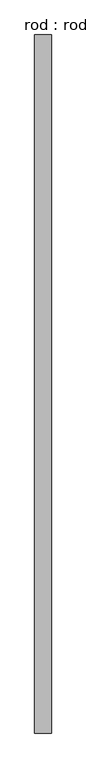
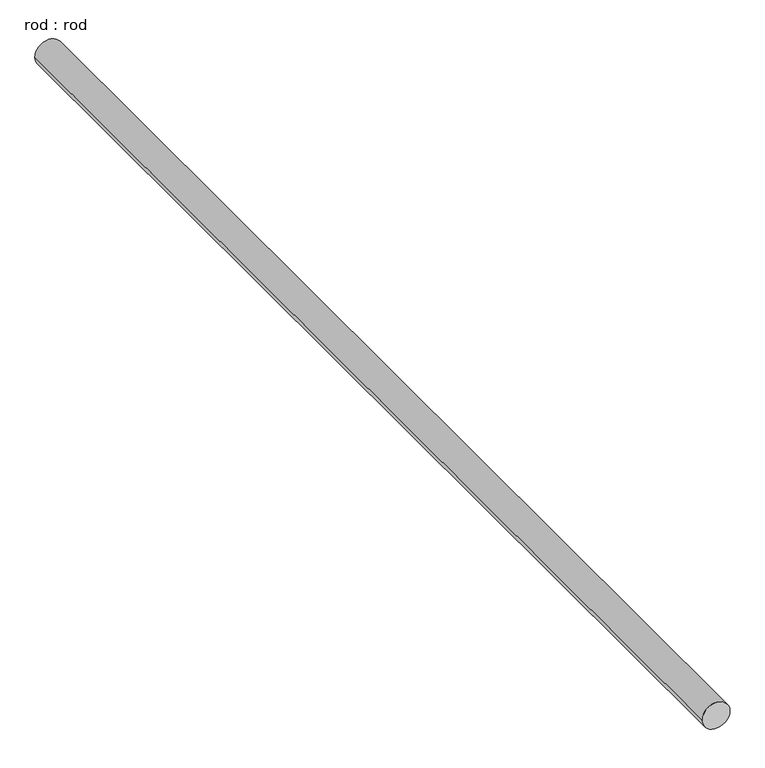
"""IFC4 building model written with IfcOpenShell, lengths in millimetres: proxy geometry, rod : rod."""

import ifcopenshell
import ifcopenshell.guid

model = None  # the IFC model being written
_history = None  # IfcOwnerHistory: only IFC2X3 demands one
_inside = {}  # id of a spatial element -> (the spatial element, [elements in it])
_under = {}  # id of a project, library or spatial element -> (it, [spatial elements below it])
_declared = {}  # id of a project -> (the project, [libraries it declares])
_typed = {}  # id of a type object -> (the type object, [elements of that type])
_made_of = {}  # id of a material, layer set ... -> (it, [elements and type objects made of it])


def new_model(schema):
    """Start an empty IFC model of exactly this schema.

    Asked for "IFC4X3", IfcOpenShell would pick the latest addendum, in which some entities
    have other attributes; the version numbers below select the first issue.
    IFC2X3 requires an IfcOwnerHistory on every rooted entity: one is made here for all.
    """
    global model, _history
    if schema == "IFC4X3":
        model = ifcopenshell.file(schema_version=(4, 3, 0, 0))
    else:
        model = ifcopenshell.file(schema=schema)
    _inside.clear()
    _under.clear()
    _declared.clear()
    _typed.clear()
    _made_of.clear()
    _history = None
    if model.schema == "IFC2X3":
        org = make("IfcOrganization", Name="unknown")
        user = make(
            "IfcPersonAndOrganization",
            ThePerson=make("IfcPerson", FamilyName="unknown"),
            TheOrganization=org,
        )
        app = make(
            "IfcApplication",
            ApplicationDeveloper=org,
            Version="unknown",
            ApplicationFullName="unknown",
            ApplicationIdentifier="unknown",
        )
        _history = make(
            "IfcOwnerHistory",
            OwningUser=user,
            OwningApplication=app,
            ChangeAction="ADDED",
            CreationDate=0,
        )
    return model


def make(cls, **values):
    """One entity of the class cls with the attributes given. An attribute that is None is left unset."""
    return model.create_entity(
        cls, **{name: value for name, value in values.items() if value is not None}
    )


def rooted(cls, **values):
    """An entity with a GlobalId (a new one), such as an element, a storey or a relation."""
    return make(cls, GlobalId=ifcopenshell.guid.new(), OwnerHistory=_history, **values)


def si_unit(unit_type, name, prefix=None):
    """IfcSIUnit, for example si_unit("LENGTHUNIT", "METRE", prefix="MILLI")."""
    return make("IfcSIUnit", UnitType=unit_type, Prefix=prefix, Name=name)


def assignment(units):
    """IfcUnitAssignment: the units of a project."""
    return None if units is None else make("IfcUnitAssignment", Units=units)


def point(xyz):
    """IfcCartesianPoint."""
    return None if xyz is None else make("IfcCartesianPoint", Coordinates=xyz)


def direction(xyz):
    """IfcDirection."""
    return None if xyz is None else make("IfcDirection", DirectionRatios=xyz)


def frame(location, z_axis=None, x_axis=None):
    """IfcAxis2Placement3D, a coordinate frame: its origin and axes. An axis left out is left unset."""
    return make(
        "IfcAxis2Placement3D",
        Location=point(location),
        Axis=direction(z_axis),
        RefDirection=direction(x_axis),
    )


def frame_2d(location, x_axis=None):
    """IfcAxis2Placement2D, a coordinate frame in the plane: its origin and x axis."""
    return make(
        "IfcAxis2Placement2D", Location=point(location), RefDirection=direction(x_axis)
    )


def origin():
    """The frame at (0, 0, 0) with its axes left unset."""
    return frame((0.0, 0.0, 0.0))


def place(relative_to, where):
    """IfcLocalPlacement: puts the frame where relative to a parent placement (None: the world)."""
    return make(
        "IfcLocalPlacement", PlacementRelTo=relative_to, RelativePlacement=where
    )


def context(
    kind, dimensions, precision=None, world=None, true_north=None, identifier=None
):
    """IfcGeometricRepresentationContext, for example the 3D "Model" context."""
    return make(
        "IfcGeometricRepresentationContext",
        ContextIdentifier=identifier,
        ContextType=kind,
        CoordinateSpaceDimension=dimensions,
        Precision=precision,
        WorldCoordinateSystem=world,
        TrueNorth=true_north,
    )


def project(units=None, contexts=None):
    """IfcProject with its units and contexts."""
    return rooted(
        "IfcProject",
        Name="project",
        RepresentationContexts=contexts,
        UnitsInContext=assignment(units),
    )


def spatial(cls, under=None, at=None, **own):
    """A site, building, storey or space (cls), placed at a placement, below another one or the project."""
    s = rooted(cls, ObjectPlacement=at, **own)
    if under is not None:
        _under.setdefault(under.id(), (under, []))[1].append(s)
    return s


def circle_curve(where, radius):
    """IfcCircle in the frame where."""
    return make("IfcCircle", Position=where, Radius=radius)


def trimmed(basis, trim1, trim2, sense, master):
    """IfcTrimmedCurve: the piece of a basis curve between two trims."""
    return make(
        "IfcTrimmedCurve",
        BasisCurve=basis,
        Trim1=trim1,
        Trim2=trim2,
        SenseAgreement=sense,
        MasterRepresentation=master,
    )


def segment(curve, same_sense, transition):
    """IfcCompositeCurveSegment."""
    return make(
        "IfcCompositeCurveSegment",
        Transition=transition,
        SameSense=same_sense,
        ParentCurve=curve,
    )


def composite_curve(segments, self_intersect=None):
    """IfcCompositeCurve: segments joined end to end."""
    return make("IfcCompositeCurve", Segments=segments, SelfIntersect=self_intersect)


def outline(outer, holes=None, kind="AREA"):
    """IfcArbitraryClosedProfileDef: a profile drawn as a closed curve; with holes, ...WithVoids."""
    if holes is None:
        return make("IfcArbitraryClosedProfileDef", ProfileType=kind, OuterCurve=outer)
    return make(
        "IfcArbitraryProfileDefWithVoids",
        ProfileType=kind,
        OuterCurve=outer,
        InnerCurves=holes,
    )


def extrude(swept, where, along, depth):
    """IfcExtrudedAreaSolid: the profile swept, set in the frame where, extruded along a direction by depth."""
    return make(
        "IfcExtrudedAreaSolid",
        SweptArea=swept,
        Position=where,
        ExtrudedDirection=direction(along),
        Depth=depth,
    )


def shape(context_of_items, identifier, shape_type, items):
    """IfcShapeRepresentation: the items that make up one representation, for example the "Body"."""
    return make(
        "IfcShapeRepresentation",
        ContextOfItems=context_of_items,
        RepresentationIdentifier=identifier,
        RepresentationType=shape_type,
        Items=items,
    )


def source(mapping_origin, context_of_items, identifier, shape_type, items):
    """IfcRepresentationMap: a shape defined once, which mapped items show again and again."""
    return make(
        "IfcRepresentationMap",
        MappingOrigin=mapping_origin,
        MappedRepresentation=shape(context_of_items, identifier, shape_type, items),
    )


def transform(
    local_origin,
    x_axis=None,
    y_axis=None,
    z_axis=None,
    scale=None,
    scale2=None,
    scale3=None,
    uniform=True,
):
    """IfcCartesianTransformationOperator3D, or its non-uniform kind. x_axis, y_axis, z_axis: its Axis1, 2, 3."""
    if uniform:
        return make(
            "IfcCartesianTransformationOperator3D",
            Axis1=direction(x_axis),
            Axis2=direction(y_axis),
            LocalOrigin=point(local_origin),
            Scale=scale,
            Axis3=direction(z_axis),
        )
    return make(
        "IfcCartesianTransformationOperator3DnonUniform",
        Axis1=direction(x_axis),
        Axis2=direction(y_axis),
        LocalOrigin=point(local_origin),
        Scale=scale,
        Axis3=direction(z_axis),
        Scale2=scale2,
        Scale3=scale3,
    )


def mapped(mapping_source, mapping_target):
    """IfcMappedItem: shows the shape of a source again, moved by a transform."""
    return make(
        "IfcMappedItem", MappingSource=mapping_source, MappingTarget=mapping_target
    )


def made_of(thing, what):
    """Note that an element or type object is made of a material, layer set ...; save() writes the relation."""
    if what is not None:
        _made_of.setdefault(what.id(), (what, []))[1].append(thing)
    return thing


def element(
    cls,
    number,
    at=None,
    inside=None,
    cuts=None,
    type_object=None,
    material=None,
    context=None,
    identifier="Body",
    shape_type=None,
    held_by="IfcProductDefinitionShape",
    body=None,
    shapes=None,
    **own,
):
    """One element of the class cls, such as IfcWall. Its Tag is "e" and its number.

    at: its placement. inside: the storey or other place that contains it. cuts: it is an
    opening in that element (IfcRelVoidsElement). A single representation is given by context,
    identifier, shape_type and body (its items); several are given by shapes. held_by: the class
    of the entity that holds the representations. save() writes the other relations.
    """
    e = rooted(cls, Tag="e%d" % number, ObjectPlacement=at, **own)
    if body is not None:
        shapes = [shape(context, identifier, shape_type, body)]
    if shapes is not None:
        e.Representation = make(held_by, Representations=shapes)
    if inside is not None:
        _inside.setdefault(inside.id(), (inside, []))[1].append(e)
    if cuts is not None:
        rooted(
            "IfcRelVoidsElement", RelatingBuildingElement=cuts, RelatedOpeningElement=e
        )
    if type_object is not None:
        _typed.setdefault(type_object.id(), (type_object, []))[1].append(e)
    return made_of(e, material)


def aggregate(whole, parts):
    """IfcRelAggregates: a whole, such as a stair, and the parts it consists of."""
    return rooted("IfcRelAggregates", RelatingObject=whole, RelatedObjects=parts)


def save(model, path):
    """Write the relations noted so far, then the file.

    IfcRelAggregates (storeys below a building ...), IfcRelContainedInSpatialStructure (elements
    in a storey), IfcRelDefinesByType, IfcRelAssociatesMaterial and IfcRelDeclares: one each for
    every whole, place, type object, material and project.
    """
    for whole, parts in _under.values():
        aggregate(whole, parts)
    for where, things in _inside.values():
        rooted(
            "IfcRelContainedInSpatialStructure",
            RelatedElements=things,
            RelatingStructure=where,
        )
    for kind, things in _typed.values():
        rooted("IfcRelDefinesByType", RelatedObjects=things, RelatingType=kind)
    for what, things in _made_of.values():
        rooted("IfcRelAssociatesMaterial", RelatedObjects=things, RelatingMaterial=what)
    for by, libraries in _declared.values():
        rooted("IfcRelDeclares", RelatingContext=by, RelatedDefinitions=libraries)
    model.write(path)


def rod_rod_3e6197a7(model_context):
    return source(origin(), model_context, "Body", "SweptSolid", [
        extrude(outline(composite_curve([segment(trimmed(circle_curve(frame_2d((0.0108462, 0.0)), 200.0), [point((0.0108462, 200.0))], [point((0.0108462, -200.0))], False, "CARTESIAN"), True, "CONTINUOUS"), segment(trimmed(circle_curve(frame_2d((0.0108462, 0.0)), 200.0), [point((0.0108462, -200.0))], [point((0.0108462, 200.0))], False, "CARTESIAN"), True, "CONTINUOUS")], self_intersect=False)), frame((0.0, -4282.9639033, 0.0), z_axis=(0.0, 1.0, 0.0), x_axis=(0.0, 0.0, 1.0)), (0.0, 0.0, 1.0), 16751.3850374),
    ])


if __name__ == "__main__":
    model = new_model("IFC4")
    model_context = context("Model", 3, world=origin())
    ifc_project = project(units=[si_unit("LENGTHUNIT", "METRE", prefix="MILLI")], contexts=[model_context])
    site = spatial("IfcSite", under=ifc_project)
    building = spatial("IfcBuilding", under=site)
    placement = place(None, origin())
    rod_rod_shape = rod_rod_3e6197a7(model_context)
    element("IfcBuildingElementProxy", 1, Name="rod : rod", ObjectType="rod : rod", at=placement, inside=building, context=model_context, shape_type="MappedRepresentation", body=[
        mapped(rod_rod_shape, transform((0.0, 0.0, 0.0), x_axis=(1.0, 0.0, 0.0), y_axis=(0.0, 1.0, 0.0), z_axis=(0.0, 0.0, 1.0))),
    ])
    save(model, "model.ifc")

# Revit data of these elements
# Type "rod : rod"
#   Default Elevation = 0
